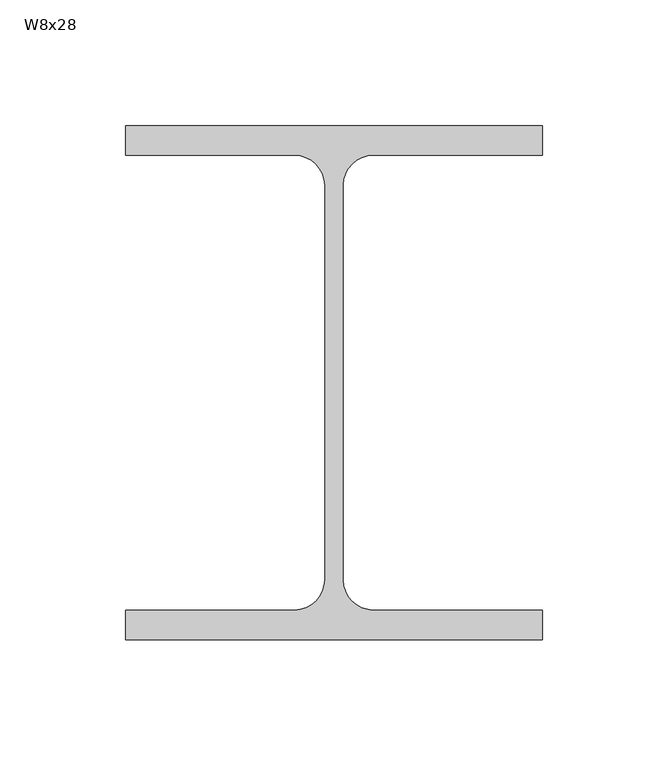
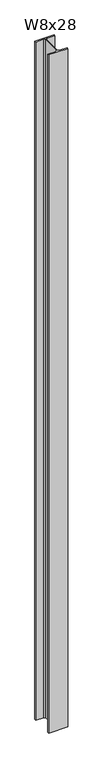
"""IFC4 building model written with IfcOpenShell, lengths in millimetres: column geometry, RME WF - Column : W8x28."""

from ifc_helpers import new_model, si_unit, point, frame, frame_2d, origin, place, context, project, spatial, polyline, circle_curve, trimmed, segment, composite_curve, outline, extrude, source, transform, mapped, element, save


def w8x28_fbbe404c(model_context):
    return source(origin(), model_context, "Body", "SweptSolid", [
        extrude(outline(composite_curve([segment(polyline([(83.058, 102.362), (83.058, 90.551), (15.621, 90.551)]), True, "CONTINUOUS"), segment(trimmed(circle_curve(frame_2d((15.621, 78.5495)), 12.0015), [point((15.621, 90.551))], [point((3.6195, 78.5495))], True, "CARTESIAN"), True, "CONTINUOUS"), segment(polyline([(3.6195, 78.5495), (3.6195, -78.5495)]), True, "CONTINUOUS"), segment(trimmed(circle_curve(frame_2d((15.621, -78.5495)), 12.0015), [point((3.6195, -78.5495))], [point((15.621, -90.551))], True, "CARTESIAN"), True, "CONTINUOUS"), segment(polyline([(15.621, -90.551), (83.058, -90.551), (83.058, -102.362), (-83.058, -102.362), (-83.058, -90.551), (-15.621, -90.551)]), True, "CONTINUOUS"), segment(trimmed(circle_curve(frame_2d((-15.621, -78.5495)), 12.0015), [point((-15.621, -90.551))], [point((-3.6195, -78.5495))], True, "CARTESIAN"), True, "CONTINUOUS"), segment(polyline([(-3.6195, -78.5495), (-3.6195, 78.5495)]), True, "CONTINUOUS"), segment(trimmed(circle_curve(frame_2d((-15.621, 78.5495)), 12.0015), [point((-3.6195, 78.5495))], [point((-15.621, 90.551))], True, "CARTESIAN"), True, "CONTINUOUS"), segment(polyline([(-15.621, 90.551), (-83.058, 90.551), (-83.058, 102.362), (83.058, 102.362)]), True, "CONTINUOUS")], self_intersect=False)), frame((0.0, 0.0, -304.8), z_axis=(0.0, 0.0, 1.0), x_axis=(1.0, 0.0, 0.0)), (0.0, 0.0, 1.0), 6172.2),
    ])


if __name__ == "__main__":
    model = new_model("IFC4")
    model_context = context("Model", 3, world=origin())
    ifc_project = project(units=[si_unit("LENGTHUNIT", "METRE", prefix="MILLI")], contexts=[model_context])
    site = spatial("IfcSite", under=ifc_project)
    building = spatial("IfcBuilding", under=site)
    placement = place(None, origin())
    w8x28_shape = w8x28_fbbe404c(model_context)
    element("IfcColumn", 1, ObjectType="RME WF - Column : W8x28", at=placement, inside=building, context=model_context, shape_type="MappedRepresentation", body=[
        mapped(w8x28_shape, transform((0.0, 0.0, 0.0), x_axis=(1.0, 0.0, 0.0), y_axis=(0.0, 1.0, 0.0), z_axis=(0.0, 0.0, 1.0))),
    ])
    save(model, "model.ifc")

# Revit data of these elements
# Type "RME WF - Column : W8x28"
#   REINF TYPE [instance default] = ""
#   Nominal Size = "W16"
#   COL REMARKS [instance default] = ""
#   BP [instance default] = ""
#   Assembly Code = "B10"
#   W = 28
#   bf = 0' - 6.54"
#   d = 0' - 8.06"
#   k = 0' - 0 15/16"
#   kr = 0' - 0.4725"
#   tf = 0' - 0.465"
#   tw = 0' - 0.285"
#   A = 0.0572222 SF
#   Structural Material [instance default] = Metal - Steel - ASTM A992
# Element 1 (IfcColumn, "RME WF - Column : W8x28")
#   Materials on its faces: "Metal - Steel - ASTM A992"
# Materials
#   "Metal - Steel - ASTM A992": class "Metal", colour RGB 255 128 0, transparency 0
